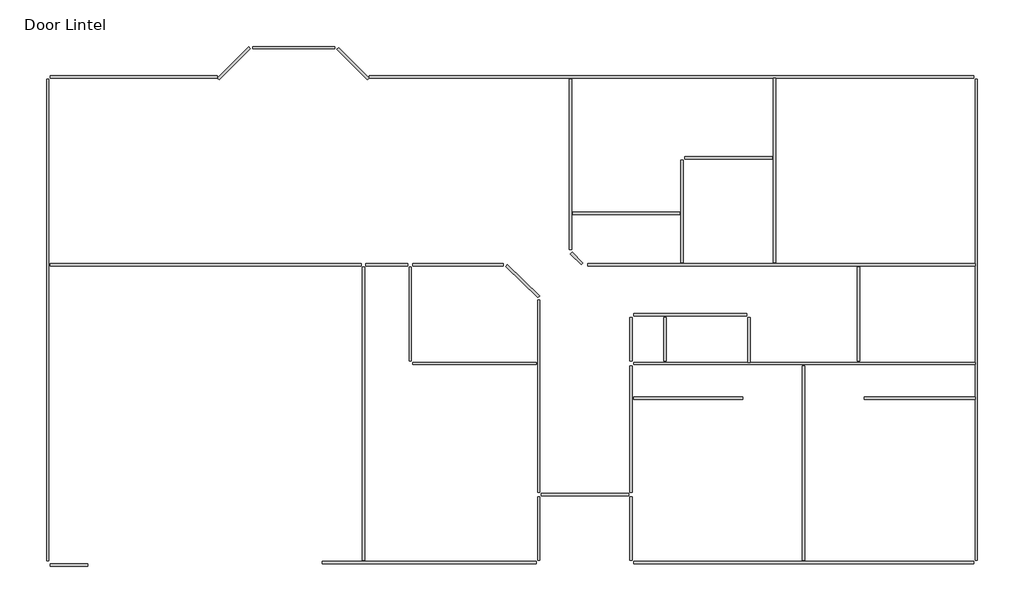
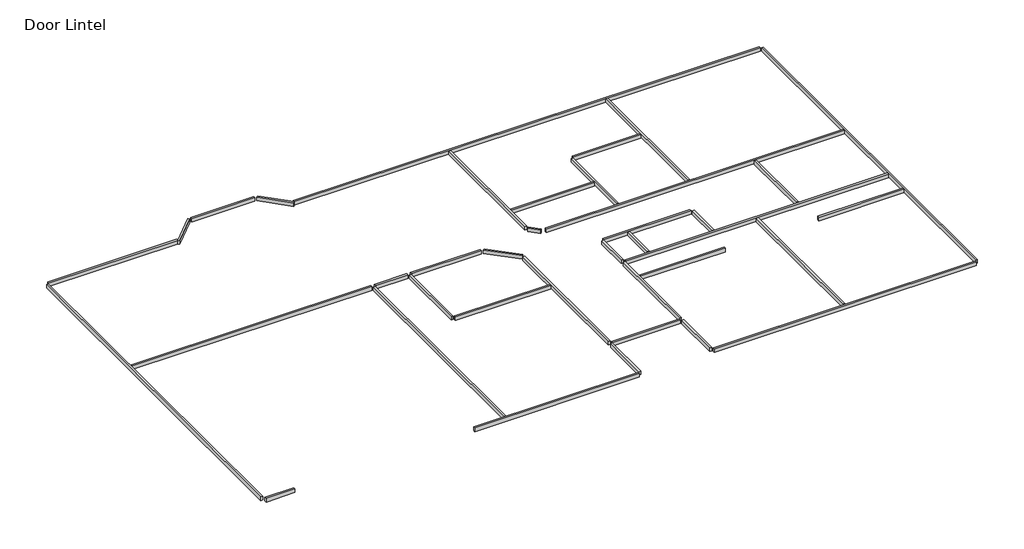
# One storey: 38 beams.
"""IFC4 building model written with IfcOpenShell, lengths in millimetres."""

import ifcopenshell
import ifcopenshell.guid

model = None  # the IFC model being written
_history = None  # IfcOwnerHistory: only IFC2X3 demands one
_inside = {}  # id of a spatial element -> (the spatial element, [elements in it])
_under = {}  # id of a project, library or spatial element -> (it, [spatial elements below it])
_declared = {}  # id of a project -> (the project, [libraries it declares])
_typed = {}  # id of a type object -> (the type object, [elements of that type])
_made_of = {}  # id of a material, layer set ... -> (it, [elements and type objects made of it])


def new_model(schema):
    """Start an empty IFC model of exactly this schema.

    Asked for "IFC4X3", IfcOpenShell would pick the latest addendum, in which some entities
    have other attributes; the version numbers below select the first issue.
    IFC2X3 requires an IfcOwnerHistory on every rooted entity: one is made here for all.
    """
    global model, _history
    if schema == "IFC4X3":
        model = ifcopenshell.file(schema_version=(4, 3, 0, 0))
    else:
        model = ifcopenshell.file(schema=schema)
    _inside.clear()
    _under.clear()
    _declared.clear()
    _typed.clear()
    _made_of.clear()
    _history = None
    if model.schema == "IFC2X3":
        org = make("IfcOrganization", Name="unknown")
        user = make(
            "IfcPersonAndOrganization",
            ThePerson=make("IfcPerson", FamilyName="unknown"),
            TheOrganization=org,
        )
        app = make(
            "IfcApplication",
            ApplicationDeveloper=org,
            Version="unknown",
            ApplicationFullName="unknown",
            ApplicationIdentifier="unknown",
        )
        _history = make(
            "IfcOwnerHistory",
            OwningUser=user,
            OwningApplication=app,
            ChangeAction="ADDED",
            CreationDate=0,
        )
    return model


def make(cls, **values):
    """One entity of the class cls with the attributes given. An attribute that is None is left unset."""
    return model.create_entity(
        cls, **{name: value for name, value in values.items() if value is not None}
    )


def rooted(cls, **values):
    """An entity with a GlobalId (a new one), such as an element, a storey or a relation."""
    return make(cls, GlobalId=ifcopenshell.guid.new(), OwnerHistory=_history, **values)


def si_unit(unit_type, name, prefix=None):
    """IfcSIUnit, for example si_unit("LENGTHUNIT", "METRE", prefix="MILLI")."""
    return make("IfcSIUnit", UnitType=unit_type, Prefix=prefix, Name=name)


def assignment(units):
    """IfcUnitAssignment: the units of a project."""
    return None if units is None else make("IfcUnitAssignment", Units=units)


def point(xyz):
    """IfcCartesianPoint."""
    return None if xyz is None else make("IfcCartesianPoint", Coordinates=xyz)


def direction(xyz):
    """IfcDirection."""
    return None if xyz is None else make("IfcDirection", DirectionRatios=xyz)


def frame(location, z_axis=None, x_axis=None):
    """IfcAxis2Placement3D, a coordinate frame: its origin and axes. An axis left out is left unset."""
    return make(
        "IfcAxis2Placement3D",
        Location=point(location),
        Axis=direction(z_axis),
        RefDirection=direction(x_axis),
    )


def origin():
    """The frame at (0, 0, 0) with its axes left unset."""
    return frame((0.0, 0.0, 0.0))


def place(relative_to, where):
    """IfcLocalPlacement: puts the frame where relative to a parent placement (None: the world)."""
    return make(
        "IfcLocalPlacement", PlacementRelTo=relative_to, RelativePlacement=where
    )


def context(
    kind, dimensions, precision=None, world=None, true_north=None, identifier=None
):
    """IfcGeometricRepresentationContext, for example the 3D "Model" context."""
    return make(
        "IfcGeometricRepresentationContext",
        ContextIdentifier=identifier,
        ContextType=kind,
        CoordinateSpaceDimension=dimensions,
        Precision=precision,
        WorldCoordinateSystem=world,
        TrueNorth=true_north,
    )


def project(units=None, contexts=None):
    """IfcProject with its units and contexts."""
    return rooted(
        "IfcProject",
        Name="project",
        RepresentationContexts=contexts,
        UnitsInContext=assignment(units),
    )


def spatial(cls, under=None, at=None, **own):
    """A site, building, storey or space (cls), placed at a placement, below another one or the project."""
    s = rooted(cls, ObjectPlacement=at, **own)
    if under is not None:
        _under.setdefault(under.id(), (under, []))[1].append(s)
    return s


def polyline(points):
    """IfcPolyline through the points."""
    return make("IfcPolyline", Points=[point(p) for p in points])


def outline(outer, holes=None, kind="AREA"):
    """IfcArbitraryClosedProfileDef: a profile drawn as a closed curve; with holes, ...WithVoids."""
    if holes is None:
        return make("IfcArbitraryClosedProfileDef", ProfileType=kind, OuterCurve=outer)
    return make(
        "IfcArbitraryProfileDefWithVoids",
        ProfileType=kind,
        OuterCurve=outer,
        InnerCurves=holes,
    )


def extrude(swept, where, along, depth):
    """IfcExtrudedAreaSolid: the profile swept, set in the frame where, extruded along a direction by depth."""
    return make(
        "IfcExtrudedAreaSolid",
        SweptArea=swept,
        Position=where,
        ExtrudedDirection=direction(along),
        Depth=depth,
    )


def shape(context_of_items, identifier, shape_type, items):
    """IfcShapeRepresentation: the items that make up one representation, for example the "Body"."""
    return make(
        "IfcShapeRepresentation",
        ContextOfItems=context_of_items,
        RepresentationIdentifier=identifier,
        RepresentationType=shape_type,
        Items=items,
    )


def source(mapping_origin, context_of_items, identifier, shape_type, items):
    """IfcRepresentationMap: a shape defined once, which mapped items show again and again."""
    return make(
        "IfcRepresentationMap",
        MappingOrigin=mapping_origin,
        MappedRepresentation=shape(context_of_items, identifier, shape_type, items),
    )


def transform(
    local_origin,
    x_axis=None,
    y_axis=None,
    z_axis=None,
    scale=None,
    scale2=None,
    scale3=None,
    uniform=True,
):
    """IfcCartesianTransformationOperator3D, or its non-uniform kind. x_axis, y_axis, z_axis: its Axis1, 2, 3."""
    if uniform:
        return make(
            "IfcCartesianTransformationOperator3D",
            Axis1=direction(x_axis),
            Axis2=direction(y_axis),
            LocalOrigin=point(local_origin),
            Scale=scale,
            Axis3=direction(z_axis),
        )
    return make(
        "IfcCartesianTransformationOperator3DnonUniform",
        Axis1=direction(x_axis),
        Axis2=direction(y_axis),
        LocalOrigin=point(local_origin),
        Scale=scale,
        Axis3=direction(z_axis),
        Scale2=scale2,
        Scale3=scale3,
    )


def mapped(mapping_source, mapping_target):
    """IfcMappedItem: shows the shape of a source again, moved by a transform."""
    return make(
        "IfcMappedItem", MappingSource=mapping_source, MappingTarget=mapping_target
    )


def made_of(thing, what):
    """Note that an element or type object is made of a material, layer set ...; save() writes the relation."""
    if what is not None:
        _made_of.setdefault(what.id(), (what, []))[1].append(thing)
    return thing


def element(
    cls,
    number,
    at=None,
    inside=None,
    cuts=None,
    type_object=None,
    material=None,
    context=None,
    identifier="Body",
    shape_type=None,
    held_by="IfcProductDefinitionShape",
    body=None,
    shapes=None,
    **own,
):
    """One element of the class cls, such as IfcWall. Its Tag is "e" and its number.

    at: its placement. inside: the storey or other place that contains it. cuts: it is an
    opening in that element (IfcRelVoidsElement). A single representation is given by context,
    identifier, shape_type and body (its items); several are given by shapes. held_by: the class
    of the entity that holds the representations. save() writes the other relations.
    """
    e = rooted(cls, Tag="e%d" % number, ObjectPlacement=at, **own)
    if body is not None:
        shapes = [shape(context, identifier, shape_type, body)]
    if shapes is not None:
        e.Representation = make(held_by, Representations=shapes)
    if inside is not None:
        _inside.setdefault(inside.id(), (inside, []))[1].append(e)
    if cuts is not None:
        rooted(
            "IfcRelVoidsElement", RelatingBuildingElement=cuts, RelatedOpeningElement=e
        )
    if type_object is not None:
        _typed.setdefault(type_object.id(), (type_object, []))[1].append(e)
    return made_of(e, material)


def aggregate(whole, parts):
    """IfcRelAggregates: a whole, such as a stair, and the parts it consists of."""
    return rooted("IfcRelAggregates", RelatingObject=whole, RelatedObjects=parts)


def save(model, path):
    """Write the relations noted so far, then the file.

    IfcRelAggregates (storeys below a building ...), IfcRelContainedInSpatialStructure (elements
    in a storey), IfcRelDefinesByType, IfcRelAssociatesMaterial and IfcRelDeclares: one each for
    every whole, place, type object, material and project.
    """
    for whole, parts in _under.values():
        aggregate(whole, parts)
    for where, things in _inside.values():
        rooted(
            "IfcRelContainedInSpatialStructure",
            RelatedElements=things,
            RelatingStructure=where,
        )
    for kind, things in _typed.values():
        rooted("IfcRelDefinesByType", RelatedObjects=things, RelatingType=kind)
    for what, things in _made_of.values():
        rooted("IfcRelAssociatesMaterial", RelatedObjects=things, RelatingMaterial=what)
    for by, libraries in _declared.values():
        rooted("IfcRelDeclares", RelatingContext=by, RelatedDefinitions=libraries)
    model.write(path)


def beam_717df711(model_context):
    return source(origin(), model_context, "Body", "SweptSolid", [
        extrude(outline(polyline([(1716.6789755, 25.4), (1716.6789755, -25.4), (-1777.9999994, -25.4), (-1777.9999994, 25.4), (1716.6789755, 25.4)])), frame((0.0, 0.0, -50.8), z_axis=(0.0, 0.0, 1.0), x_axis=(1.0, 0.0, 0.0)), (0.0, 0.0, 1.0), 101.6),
    ])


def beam_0fe92c09(model_context):
    return source(origin(), model_context, "Body", "SweptSolid", [
        extrude(outline(polyline([(431.690501, 25.4), (431.690501, -25.4), (-492.3733183, -25.4), (-492.3733183, 25.4), (431.690501, 25.4)])), frame((0.0, 0.0, -50.8), z_axis=(0.0, 0.0, 1.0), x_axis=(1.0, 0.0, 0.0)), (0.0, 0.0, 1.0), 101.6),
    ])


def beam_3500c81b(model_context):
    return source(origin(), model_context, "Body", "SweptSolid", [
        extrude(outline(polyline([(863.6, 25.4), (863.6, -25.4), (-845.1882072, -25.4), (-845.1882072, 25.4), (863.6, 25.4)])), frame((0.0, 0.0, -50.8), z_axis=(0.0, 0.0, 1.0), x_axis=(1.0, 0.0, 0.0)), (0.0, 0.0, 1.0), 101.6),
    ])


def beam_4e9e3d70(model_context):
    return source(origin(), model_context, "Body", "SweptSolid", [
        extrude(outline(polyline([(492.3733183, 25.4), (492.3733183, -25.4), (-405.6522938, -25.4), (-405.6522938, 25.4), (492.3733183, 25.4)])), frame((0.0, 0.0, -50.8), z_axis=(0.0, 0.0, 1.0), x_axis=(1.0, 0.0, 0.0)), (0.0, 0.0, 1.0), 101.6),
    ])


def beam_5a8d2df6(model_context):
    return source(origin(), model_context, "Body", "SweptSolid", [
        extrude(outline(polyline([(6349.9999994, 25.4), (6349.9999994, -25.4), (-6288.6789755, -25.4), (-6288.6789755, 25.4), (6349.9999994, 25.4)])), frame((0.0, 0.0, -50.8), z_axis=(0.0, 0.0, 1.0), x_axis=(1.0, 0.0, 0.0)), (0.0, 0.0, 1.0), 101.6),
    ])


def beam_8dd97a7c(model_context):
    return source(origin(), model_context, "Body", "SweptSolid", [
        extrude(outline(polyline([(5029.1999994, 25.4), (5029.1999994, -25.4), (-5029.1999994, -25.4), (-5029.1999994, 25.4), (5029.1999994, 25.4)])), frame((0.0, 0.0, -50.8), z_axis=(0.0, 0.0, 1.0), x_axis=(1.0, 0.0, 0.0)), (0.0, 0.0, 1.0), 101.6),
    ])


def beam_44bcd8c2(model_context):
    return source(origin(), model_context, "Body", "SweptSolid", [
        extrude(outline(polyline([(3555.9999994, 25.4), (3555.9999994, -25.4), (-3555.9999994, -25.4), (-3555.9999994, 25.4), (3555.9999994, 25.4)])), frame((0.0, 0.0, -50.8), z_axis=(0.0, 0.0, 1.0), x_axis=(1.0, 0.0, 0.0)), (0.0, 0.0, 1.0), 101.6),
    ])


def beam_ec20356b(model_context):
    return source(origin(), model_context, "Body", "SweptSolid", [
        extrude(outline(polyline([(660.3999994, 25.4), (660.3999994, -25.4), (-660.3999994, -25.4), (-660.3999994, 25.4), (660.3999994, 25.4)])), frame((0.0, 0.0, -50.8), z_axis=(0.0, 0.0, 1.0), x_axis=(1.0, 0.0, 0.0)), (0.0, 0.0, 1.0), 101.6),
    ])


def beam_17170791(model_context):
    return source(origin(), model_context, "Body", "SweptSolid", [
        extrude(outline(polyline([(914.3999994, 25.4), (914.3999994, -25.4), (-914.3999994, -25.4), (-914.3999994, 25.4), (914.3999994, 25.4)])), frame((0.0, 0.0, -50.8), z_axis=(0.0, 0.0, 1.0), x_axis=(1.0, 0.0, 0.0)), (0.0, 0.0, 1.0), 101.6),
    ])


def beam_5c93efd5(model_context):
    return source(origin(), model_context, "Body", "SweptSolid", [
        extrude(outline(polyline([(3063.8749994, 25.4), (3063.8749994, -25.4), (-3063.8749994, -25.4), (-3063.8749994, 25.4), (3063.8749994, 25.4)])), frame((0.0, 0.0, -50.8), z_axis=(0.0, 0.0, 1.0), x_axis=(1.0, 0.0, 0.0)), (0.0, 0.0, 1.0), 101.6),
    ])


def beam_4ff5e491(model_context):
    return source(origin(), model_context, "Body", "SweptSolid", [
        extrude(outline(polyline([(3248.0249994, 25.4), (3248.0249994, -25.4), (-3248.0249994, -25.4), (-3248.0249994, 25.4), (3248.0249994, 25.4)])), frame((0.0, 0.0, -50.8), z_axis=(0.0, 0.0, 1.0), x_axis=(1.0, 0.0, 0.0)), (0.0, 0.0, 1.0), 101.6),
    ])


def beam_e0e1cdb9(model_context):
    return source(origin(), model_context, "Body", "SweptSolid", [
        extrude(outline(polyline([(444.5, 25.4), (444.5, -25.4), (-431.7999994, -25.4), (-431.7999994, 25.4), (444.5, 25.4)])), frame((0.0, 0.0, -50.8), z_axis=(0.0, 0.0, 1.0), x_axis=(1.0, 0.0, 0.0)), (0.0, 0.0, 1.0), 101.6),
    ])


def beam_a7f65a44(model_context):
    return source(origin(), model_context, "Body", "SweptSolid", [
        extrude(outline(polyline([(921.932951, 25.4), (921.932951, -25.4), (-972.7329504, -25.4), (-972.7329504, 25.4), (921.932951, 25.4)])), frame((0.0, 0.0, -50.8), z_axis=(0.0, 0.0, 1.0), x_axis=(1.0, 0.0, 0.0)), (0.0, 0.0, 1.0), 101.6),
    ])


def beam_c7262e2a(model_context):
    return source(origin(), model_context, "Body", "SweptSolid", [
        extrude(outline(polyline([(450.6043361, 25.4), (450.6043361, -25.4), (-488.5308943, -25.4), (-488.5308943, 25.4), (450.6043361, 25.4)])), frame((0.0, 0.0, -50.8), z_axis=(0.0, 0.0, 1.0), x_axis=(1.0, 0.0, 0.0)), (0.0, 0.0, 1.0), 101.6),
    ])


def beam_d1363b41(model_context):
    return source(origin(), model_context, "Body", "SweptSolid", [
        extrude(outline(polyline([(1292.2249994, 25.4), (1292.2249994, -25.4), (-1292.2249994, -25.4), (-1292.2249994, 25.4), (1292.2249994, 25.4)])), frame((0.0, 0.0, -50.8), z_axis=(0.0, 0.0, 1.0), x_axis=(1.0, 0.0, 0.0)), (0.0, 0.0, 1.0), 101.6),
    ])


def beam_1eeaf63e(model_context):
    return source(origin(), model_context, "Body", "SweptSolid", [
        extrude(outline(polyline([(955.675, 25.4), (955.675, -25.4), (-1006.4749994, -25.4), (-1006.4749994, 25.4), (955.675, 25.4)])), frame((0.0, 0.0, -50.8), z_axis=(0.0, 0.0, 1.0), x_axis=(1.0, 0.0, 0.0)), (0.0, 0.0, 1.0), 101.6),
    ])


def beam_6ddf0adc(model_context):
    return source(origin(), model_context, "Body", "SweptSolid", [
        extrude(outline(polyline([(2020.4829504, 25.4), (2020.4829504, -25.4), (-1995.082951, -25.4), (-1995.082951, 25.4), (2020.4829504, 25.4)])), frame((0.0, 0.0, -50.8), z_axis=(0.0, 0.0, 1.0), x_axis=(1.0, 0.0, 0.0)), (0.0, 0.0, 1.0), 101.6),
    ])


def beam_5a6f5897(model_context):
    return source(origin(), model_context, "Body", "SweptSolid", [
        extrude(outline(polyline([(1795.057951, 25.4), (1795.057951, -25.4), (-1769.657951, -25.4), (-1769.657951, 25.4), (1795.057951, 25.4)])), frame((0.0, 0.0, -50.8), z_axis=(0.0, 0.0, 1.0), x_axis=(1.0, 0.0, 0.0)), (0.0, 0.0, 1.0), 101.6),
    ])


def beam_8933aaf6(model_context):
    return source(origin(), model_context, "Body", "SweptSolid", [
        extrude(outline(polyline([(161.5124332, 25.4), (161.5124332, -25.4), (-161.5124332, -25.4), (-161.5124332, 25.4), (161.5124332, 25.4)])), frame((0.0, 0.0, -50.8), z_axis=(0.0, 0.0, 1.0), x_axis=(1.0, 0.0, 0.0)), (0.0, 0.0, 1.0), 101.6),
    ])


def beam_50604119(model_context):
    return source(origin(), model_context, "Body", "SweptSolid", [
        extrude(outline(polyline([(1117.6, 25.4), (1117.6, -25.4), (-1117.6, -25.4), (-1117.6, 25.4), (1117.6, 25.4)])), frame((0.0, 0.0, -50.8), z_axis=(0.0, 0.0, 1.0), x_axis=(1.0, 0.0, 0.0)), (0.0, 0.0, 1.0), 101.6),
    ])


def beam_0149d91d(model_context):
    return source(origin(), model_context, "Body", "SweptSolid", [
        extrude(outline(polyline([(4058.832951, 25.4), (4058.832951, -25.4), (-4033.432951, -25.4), (-4033.432951, 25.4), (4058.832951, 25.4)])), frame((0.0, 0.0, -50.8), z_axis=(0.0, 0.0, 1.0), x_axis=(1.0, 0.0, 0.0)), (0.0, 0.0, 1.0), 101.6),
    ])


def beam_4f4e5714(model_context):
    return source(origin(), model_context, "Body", "SweptSolid", [
        extrude(outline(polyline([(1066.8, 25.4), (1066.8, -25.4), (-1066.8, -25.4), (-1066.8, 25.4), (1066.8, 25.4)])), frame((0.0, 0.0, -50.8), z_axis=(0.0, 0.0, 1.0), x_axis=(1.0, 0.0, 0.0)), (0.0, 0.0, 1.0), 101.6),
    ])


def beam_dc030418(model_context):
    return source(origin(), model_context, "Body", "SweptSolid", [
        extrude(outline(polyline([(914.4, 25.4), (914.4, -25.4), (-914.4, -25.4), (-914.4, 25.4), (914.4, 25.4)])), frame((0.0, 0.0, -50.8), z_axis=(0.0, 0.0, 1.0), x_axis=(1.0, 0.0, 0.0)), (0.0, 0.0, 1.0), 101.6),
    ])


def beam_32b3ca21(model_context):
    return source(origin(), model_context, "Body", "SweptSolid", [
        extrude(outline(polyline([(1914.525, 25.4), (1914.525, -25.4), (-1939.925, -25.4), (-1939.925, 25.4), (1914.525, 25.4)])), frame((0.0, 0.0, -50.8), z_axis=(0.0, 0.0, 1.0), x_axis=(1.0, 0.0, 0.0)), (0.0, 0.0, 1.0), 101.6),
    ])


def beam_af15350c(model_context):
    return source(origin(), model_context, "Body", "SweptSolid", [
        extrude(outline(polyline([(1181.1, 25.4), (1181.1, -25.4), (-1181.1, -25.4), (-1181.1, 25.4), (1181.1, 25.4)])), frame((0.0, 0.0, -50.8), z_axis=(0.0, 0.0, 1.0), x_axis=(1.0, 0.0, 0.0)), (0.0, 0.0, 1.0), 101.6),
    ])


def beam_60fbd3f3(model_context):
    return source(origin(), model_context, "Body", "SweptSolid", [
        extrude(outline(polyline([(457.2, 25.4), (457.2, -25.4), (-457.2, -25.4), (-457.2, 25.4), (457.2, 25.4)])), frame((0.0, 0.0, -50.8), z_axis=(0.0, 0.0, 1.0), x_axis=(1.0, 0.0, 0.0)), (0.0, 0.0, 1.0), 101.6),
    ])


def beam_38f3c654(model_context):
    return source(origin(), model_context, "Body", "SweptSolid", [
        extrude(outline(polyline([(3581.4, 25.4), (3581.4, -25.4), (-3556.0, -25.4), (-3556.0, 25.4), (3581.4, 25.4)])), frame((0.0, 0.0, -50.8), z_axis=(0.0, 0.0, 1.0), x_axis=(1.0, 0.0, 0.0)), (0.0, 0.0, 1.0), 101.6),
    ])


def beam_f72471f4(model_context):
    return source(origin(), model_context, "Body", "SweptSolid", [
        extrude(outline(polyline([(482.6, 25.4), (482.6, -25.4), (-457.2, -25.4), (-457.2, 25.4), (482.6, 25.4)])), frame((0.0, 0.0, -50.8), z_axis=(0.0, 0.0, 1.0), x_axis=(1.0, 0.0, 0.0)), (0.0, 0.0, 1.0), 101.6),
    ])


def beam_0b80d38c(model_context):
    return source(origin(), model_context, "Body", "SweptSolid", [
        extrude(outline(polyline([(1143.0, 25.4), (1143.0, -25.4), (-1143.0, -25.4), (-1143.0, 25.4), (1143.0, 25.4)])), frame((0.0, 0.0, -50.8), z_axis=(0.0, 0.0, 1.0), x_axis=(1.0, 0.0, 0.0)), (0.0, 0.0, 1.0), 101.6),
    ])


def beam_8729cf3f(model_context):
    return source(origin(), model_context, "Body", "SweptSolid", [
        extrude(outline(polyline([(981.075, 25.4), (981.075, -25.4), (-981.075, -25.4), (-981.075, 25.4), (981.075, 25.4)])), frame((0.0, 0.0, -50.8), z_axis=(0.0, 0.0, 1.0), x_axis=(1.0, 0.0, 0.0)), (0.0, 0.0, 1.0), 101.6),
    ])


def beam_71e3b4ab(model_context):
    return source(origin(), model_context, "Body", "SweptSolid", [
        extrude(outline(polyline([(1168.4, 25.4), (1168.4, -25.4), (-1143.0, -25.4), (-1143.0, 25.4), (1168.4, 25.4)])), frame((0.0, 0.0, -50.8), z_axis=(0.0, 0.0, 1.0), x_axis=(1.0, 0.0, 0.0)), (0.0, 0.0, 1.0), 101.6),
    ])


def beam_d87feb12(model_context):
    return source(origin(), model_context, "Body", "SweptSolid", [
        extrude(outline(polyline([(2032.0, 25.4), (2032.0, -25.4), (-2032.0, -25.4), (-2032.0, 25.4), (2032.0, 25.4)])), frame((0.0, 0.0, -50.8), z_axis=(0.0, 0.0, 1.0), x_axis=(1.0, 0.0, 0.0)), (0.0, 0.0, 1.0), 101.6),
    ])


def beam_35a73032(model_context):
    return source(origin(), model_context, "Body", "SweptSolid", [
        extrude(outline(polyline([(1320.8, 25.4), (1320.8, -25.4), (-1320.8, -25.4), (-1320.8, 25.4), (1320.8, 25.4)])), frame((0.0, 0.0, -50.8), z_axis=(0.0, 0.0, 1.0), x_axis=(1.0, 0.0, 0.0)), (0.0, 0.0, 1.0), 101.6),
    ])


def beam_ce158ae4(model_context):
    return source(origin(), model_context, "Body", "SweptSolid", [
        extrude(outline(polyline([(392.1124994, 25.4), (392.1124994, -25.4), (-392.1125, -25.4), (-392.1125, 25.4), (392.1124994, 25.4)])), frame((0.0, 0.0, -50.8), z_axis=(0.0, 0.0, 1.0), x_axis=(1.0, 0.0, 0.0)), (0.0, 0.0, 1.0), 101.6),
    ])


def beam_4f005310(model_context):
    return source(origin(), model_context, "Body", "SweptSolid", [
        extrude(outline(polyline([(5035.5499994, 25.4), (5035.5499994, -25.4), (-5035.55, -25.4), (-5035.55, 25.4), (5035.5499994, 25.4)])), frame((0.0, 0.0, -50.8), z_axis=(0.0, 0.0, 1.0), x_axis=(1.0, 0.0, 0.0)), (0.0, 0.0, 1.0), 101.6),
    ])


def beam_f884bc05(model_context):
    return source(origin(), model_context, "Body", "SweptSolid", [
        extrude(outline(polyline([(2235.2, 25.4), (2235.2, -25.4), (-2235.1999994, -25.4), (-2235.1999994, 25.4), (2235.2, 25.4)])), frame((0.0, 0.0, -50.8), z_axis=(0.0, 0.0, 1.0), x_axis=(1.0, 0.0, 0.0)), (0.0, 0.0, 1.0), 101.6),
    ])


model = new_model("IFC4")

# Units and contexts
model_context = context("Model", 3, world=origin())
ifc_project = project(units=[si_unit("LENGTHUNIT", "METRE", prefix="MILLI")], contexts=[model_context])

# Site, building, storey
site = spatial("IfcSite", under=ifc_project)
building = spatial("IfcBuilding", under=site)
storey = spatial("IfcBuildingStorey", under=building, Name="Door Lintel", Elevation=2387.6)

# Beams
placement = place(None, origin())
beam_shape = beam_717df711(model_context)
element("IfcBeam", 1, ObjectType="Dimension Lumber : BLDG 6241 2X4\" TRUSS MEMBER", at=placement, inside=storey, context=model_context, shape_type="MappedRepresentation", body=[
    mapped(beam_shape, transform((-15921.614829, 5156.9284114, 2336.8), x_axis=(1.0, 0.0, 0.0), y_axis=(0.0, 1.0, 0.0), z_axis=(0.0, 0.0, 1.0))),
])
beam_2_shape = beam_0fe92c09(model_context)
element("IfcBeam", 2, ObjectType="Dimension Lumber : BLDG 6241 2X4\" TRUSS MEMBER", at=placement, inside=storey, context=model_context, shape_type="MappedRepresentation", body=[
    mapped(beam_2_shape, transform((-13838.814829, 5461.7284114, 2336.8), x_axis=(0.7071067811865482, 0.7071067811865469, 0.0), y_axis=(-0.7071067811865469, 0.7071067811865482, 0.0), z_axis=(0.0, 0.0, 1.0))),
])
beam_3_shape = beam_3500c81b(model_context)
element("IfcBeam", 3, ObjectType="Dimension Lumber : BLDG 6241 2X4\" TRUSS MEMBER", at=placement, inside=storey, context=model_context, shape_type="MappedRepresentation", body=[
    mapped(beam_3_shape, transform((-12619.614829, 5766.5284114, 2336.8), x_axis=(1.0, 0.0, 0.0), y_axis=(0.0, 1.0, 0.0), z_axis=(0.0, 0.0, 1.0))),
])
beam_4_shape = beam_4e9e3d70(model_context)
element("IfcBeam", 4, ObjectType="Dimension Lumber : BLDG 6241 2X4\" TRUSS MEMBER", at=placement, inside=storey, context=model_context, shape_type="MappedRepresentation", body=[
    mapped(beam_4_shape, transform((-11400.414829, 5461.7284114, 2336.8), x_axis=(0.7071067811865464, -0.7071067811865488, 0.0), y_axis=(0.7071067811865488, 0.7071067811865464, 0.0), z_axis=(0.0, 0.0, 1.0))),
])
beam_5_shape = beam_5a8d2df6(model_context)
element("IfcBeam", 5, ObjectType="Dimension Lumber : BLDG 6241 2X4\" TRUSS MEMBER", at=placement, inside=storey, context=model_context, shape_type="MappedRepresentation", body=[
    mapped(beam_5_shape, transform((-4745.614829, 5156.9284114, 2336.8), x_axis=(1.0, 0.0, 0.0), y_axis=(0.0, 1.0, 0.0), z_axis=(0.0, 0.0, 1.0))),
])
beam_6_shape = beam_8dd97a7c(model_context)
element("IfcBeam", 6, ObjectType="Dimension Lumber : BLDG 6241 2X4\" TRUSS MEMBER", at=placement, inside=storey, context=model_context, shape_type="MappedRepresentation", body=[
    mapped(beam_6_shape, transform((1655.185171, 76.9284114, 2336.8), x_axis=(0.0, -1.0, 0.0), y_axis=(1.0, 0.0, 0.0), z_axis=(0.0, 0.0, 1.0))),
])
beam_7_shape = beam_44bcd8c2(model_context)
element("IfcBeam", 7, ObjectType="Dimension Lumber : BLDG 6241 2X4\" TRUSS MEMBER", at=placement, inside=storey, context=model_context, shape_type="MappedRepresentation", body=[
    mapped(beam_7_shape, transform((-1951.614829, -5003.0715886, 2336.8), x_axis=(-1.0, 0.0, 0.0), y_axis=(0.0, -1.0, 0.0), z_axis=(0.0, 0.0, 1.0))),
])
beam_8_shape = beam_ec20356b(model_context)
element("IfcBeam", 8, ObjectType="Dimension Lumber : BLDG 6241 2X4\" TRUSS MEMBER", at=placement, inside=storey, context=model_context, shape_type="MappedRepresentation", body=[
    mapped(beam_8_shape, transform((-5558.414829, -4291.8715886, 2336.8), x_axis=(0.0, 1.0, 0.0), y_axis=(-1.0, 0.0, 0.0), z_axis=(0.0, 0.0, 1.0))),
])
element("IfcBeam", 9, ObjectType="Dimension Lumber : BLDG 6241 2X4\" TRUSS MEMBER", at=placement, inside=storey, context=model_context, shape_type="MappedRepresentation", body=[
    mapped(beam_8_shape, transform((-7488.814829, -4291.8715886, 2336.8), x_axis=(0.0, -1.0, 0.0), y_axis=(1.0, 0.0, 0.0), z_axis=(0.0, 0.0, 1.0))),
])
beam_9_shape = beam_17170791(model_context)
element("IfcBeam", 10, ObjectType="Dimension Lumber : BLDG 6241 2X4\" TRUSS MEMBER", at=placement, inside=storey, context=model_context, shape_type="MappedRepresentation", body=[
    mapped(beam_9_shape, transform((-6523.614829, -3580.6715886, 2336.8), x_axis=(-1.0, 0.0, 0.0), y_axis=(0.0, -1.0, 0.0), z_axis=(0.0, 0.0, 1.0))),
])
beam_10_shape = beam_5c93efd5(model_context)
element("IfcBeam", 11, ObjectType="Dimension Lumber : BLDG 6241 2X4\" TRUSS MEMBER", at=placement, inside=storey, context=model_context, shape_type="MappedRepresentation", body=[
    mapped(beam_10_shape, transform((-11152.764829, -1888.3965886, 2336.8), x_axis=(0.0, 1.0, 0.0), y_axis=(-1.0, 0.0, 0.0), z_axis=(0.0, 0.0, 1.0))),
])
beam_11_shape = beam_4ff5e491(model_context)
element("IfcBeam", 12, ObjectType="Dimension Lumber : BLDG 6241 2X4\" TRUSS MEMBER", at=placement, inside=storey, context=model_context, shape_type="MappedRepresentation", body=[
    mapped(beam_11_shape, transform((-14451.589829, 1226.2784114, 2336.8), x_axis=(-1.0, 0.0, 0.0), y_axis=(0.0, -1.0, 0.0), z_axis=(0.0, 0.0, 1.0))),
])
beam_12_shape = beam_e0e1cdb9(model_context)
element("IfcBeam", 13, ObjectType="Dimension Lumber : BLDG 6241 2X4\" TRUSS MEMBER", at=placement, inside=storey, context=model_context, shape_type="MappedRepresentation", body=[
    mapped(beam_12_shape, transform((-10670.164829, 1226.2784114, 2336.8), x_axis=(1.0, 0.0, 0.0), y_axis=(0.0, 1.0, 0.0), z_axis=(0.0, 0.0, 1.0))),
])
beam_13_shape = beam_a7f65a44(model_context)
element("IfcBeam", 14, ObjectType="Dimension Lumber : BLDG 6241 2X4\" TRUSS MEMBER", at=placement, inside=storey, context=model_context, shape_type="MappedRepresentation", body=[
    mapped(beam_13_shape, transform((-9151.331878, 1226.2784114, 2336.8), x_axis=(1.0, 0.0, 0.0), y_axis=(0.0, 1.0, 0.0), z_axis=(0.0, 0.0, 1.0))),
])
beam_14_shape = beam_c7262e2a(model_context)
element("IfcBeam", 15, ObjectType="Dimension Lumber : BLDG 6241 2X4\" TRUSS MEMBER", at=placement, inside=storey, context=model_context, shape_type="MappedRepresentation", body=[
    mapped(beam_14_shape, transform((-7810.4858535, 868.6863624, 2336.8), x_axis=(0.7172827972504613, -0.6967821673726686, 0.0), y_axis=(0.6967821673726686, 0.7172827972504613, 0.0), z_axis=(0.0, 0.0, 1.0))),
])
beam_15_shape = beam_d1363b41(model_context)
element("IfcBeam", 16, ObjectType="Dimension Lumber : BLDG 6241 2X4\" TRUSS MEMBER", at=placement, inside=storey, context=model_context, shape_type="MappedRepresentation", body=[
    mapped(beam_15_shape, transform((-8831.839829, -837.4715886, 2336.8), x_axis=(1.0, 0.0, 0.0), y_axis=(0.0, 1.0, 0.0), z_axis=(0.0, 0.0, 1.0))),
])
beam_16_shape = beam_1eeaf63e(model_context)
element("IfcBeam", 17, ObjectType="Dimension Lumber : BLDG 6241 2X4\" TRUSS MEMBER", at=placement, inside=storey, context=model_context, shape_type="MappedRepresentation", body=[
    mapped(beam_16_shape, transform((-10174.864829, 219.8034114, 2336.8), x_axis=(0.0, 1.0, 0.0), y_axis=(-1.0, 0.0, 0.0), z_axis=(0.0, 0.0, 1.0))),
])
beam_17_shape = beam_6ddf0adc(model_context)
element("IfcBeam", 18, ObjectType="Dimension Lumber : BLDG 6241 2X4\" TRUSS MEMBER", at=placement, inside=storey, context=model_context, shape_type="MappedRepresentation", body=[
    mapped(beam_17_shape, transform((-7488.814829, -1509.3886376, 2336.8), x_axis=(0.0, -1.0, 0.0), y_axis=(1.0, 0.0, 0.0), z_axis=(0.0, 0.0, 1.0))),
])
beam_18_shape = beam_5a6f5897(model_context)
element("IfcBeam", 19, ObjectType="Dimension Lumber : BLDG 6241 2X4\" TRUSS MEMBER", at=placement, inside=storey, context=model_context, shape_type="MappedRepresentation", body=[
    mapped(beam_18_shape, transform((-6828.414829, 3336.4704603, 2336.8), x_axis=(0.0, -1.0, 0.0), y_axis=(1.0, 0.0, 0.0), z_axis=(0.0, 0.0, 1.0))),
])
beam_19_shape = beam_8933aaf6(model_context)
element("IfcBeam", 20, ObjectType="Dimension Lumber : BLDG 6241 2X4\" TRUSS MEMBER", at=placement, inside=storey, context=model_context, shape_type="MappedRepresentation", body=[
    mapped(beam_19_shape, transform((-6696.2477801, 1358.4454603, 2336.8), x_axis=(-0.7071067811865457, 0.7071067811865493, 0.0), y_axis=(-0.7071067811865493, -0.7071067811865457, 0.0), z_axis=(0.0, 0.0, 1.0))),
])
beam_20_shape = beam_50604119(model_context)
element("IfcBeam", 21, ObjectType="Dimension Lumber : BLDG 6241 2X4\" TRUSS MEMBER", at=placement, inside=storey, context=model_context, shape_type="MappedRepresentation", body=[
    mapped(beam_20_shape, transform((-5660.014829, 2305.7784114, 2336.8), x_axis=(1.0, 0.0, 0.0), y_axis=(0.0, 1.0, 0.0), z_axis=(0.0, 0.0, 1.0))),
])
beam_21_shape = beam_0149d91d(model_context)
element("IfcBeam", 22, ObjectType="Dimension Lumber : BLDG 6241 2X4\" TRUSS MEMBER", at=placement, inside=storey, context=model_context, shape_type="MappedRepresentation", body=[
    mapped(beam_21_shape, transform((-2429.0477801, 1226.2784114, 2336.8), x_axis=(1.0, 0.0, 0.0), y_axis=(0.0, 1.0, 0.0), z_axis=(0.0, 0.0, 1.0))),
])
beam_22_shape = beam_4f4e5714(model_context)
element("IfcBeam", 23, ObjectType="Dimension Lumber : BLDG 6241 2X4\" TRUSS MEMBER", at=placement, inside=storey, context=model_context, shape_type="MappedRepresentation", body=[
    mapped(beam_22_shape, transform((-4491.614829, 2343.8784114, 2336.8), x_axis=(0.0, 1.0, 0.0), y_axis=(-1.0, 0.0, 0.0), z_axis=(0.0, 0.0, 1.0))),
])
beam_23_shape = beam_dc030418(model_context)
element("IfcBeam", 24, ObjectType="Dimension Lumber : BLDG 6241 2X4\" TRUSS MEMBER", at=placement, inside=storey, context=model_context, shape_type="MappedRepresentation", body=[
    mapped(beam_23_shape, transform((-3526.414829, 3461.4784114, 2336.8), x_axis=(1.0, 0.0, 0.0), y_axis=(0.0, 1.0, 0.0), z_axis=(0.0, 0.0, 1.0))),
])
beam_24_shape = beam_32b3ca21(model_context)
element("IfcBeam", 25, ObjectType="Dimension Lumber : BLDG 6241 2X4\" TRUSS MEMBER", at=placement, inside=storey, context=model_context, shape_type="MappedRepresentation", body=[
    mapped(beam_24_shape, transform((-2561.214829, 3191.6034114, 2336.8), x_axis=(0.0, -1.0, 0.0), y_axis=(1.0, 0.0, 0.0), z_axis=(0.0, 0.0, 1.0))),
])
beam_25_shape = beam_af15350c(model_context)
element("IfcBeam", 26, ObjectType="Dimension Lumber : BLDG 6241 2X4\" TRUSS MEMBER", at=placement, inside=storey, context=model_context, shape_type="MappedRepresentation", body=[
    mapped(beam_25_shape, transform((-4326.514829, 178.5284114, 2336.8), x_axis=(1.0, 0.0, 0.0), y_axis=(0.0, 1.0, 0.0), z_axis=(0.0, 0.0, 1.0))),
])
beam_26_shape = beam_60fbd3f3(model_context)
element("IfcBeam", 27, ObjectType="Dimension Lumber : BLDG 6241 2X4\" TRUSS MEMBER", at=placement, inside=storey, context=model_context, shape_type="MappedRepresentation", body=[
    mapped(beam_26_shape, transform((-5558.414829, -329.4715886, 2336.8), x_axis=(0.0, 1.0, 0.0), y_axis=(-1.0, 0.0, 0.0), z_axis=(0.0, 0.0, 1.0))),
])
element("IfcBeam", 28, ObjectType="Dimension Lumber : BLDG 6241 2X4\" TRUSS MEMBER", at=placement, inside=storey, context=model_context, shape_type="MappedRepresentation", body=[
    mapped(beam_26_shape, transform((-4847.214829, -329.4715886, 2336.8), x_axis=(0.0, 1.0, 0.0), y_axis=(-1.0, 0.0, 0.0), z_axis=(0.0, 0.0, 1.0))),
])
beam_27_shape = beam_38f3c654(model_context)
element("IfcBeam", 29, ObjectType="Dimension Lumber : BLDG 6241 2X4\" TRUSS MEMBER", at=placement, inside=storey, context=model_context, shape_type="MappedRepresentation", body=[
    mapped(beam_27_shape, transform((-1951.614829, -837.4715886, 2336.8), x_axis=(1.0, 0.0, 0.0), y_axis=(0.0, 1.0, 0.0), z_axis=(0.0, 0.0, 1.0))),
])
beam_28_shape = beam_f72471f4(model_context)
element("IfcBeam", 30, ObjectType="Dimension Lumber : BLDG 6241 2X4\" TRUSS MEMBER", at=placement, inside=storey, context=model_context, shape_type="MappedRepresentation", body=[
    mapped(beam_28_shape, transform((-3094.614829, -329.4715886, 2336.8), x_axis=(0.0, -1.0, 0.0), y_axis=(1.0, 0.0, 0.0), z_axis=(0.0, 0.0, 1.0))),
])
beam_29_shape = beam_0b80d38c(model_context)
element("IfcBeam", 31, ObjectType="Dimension Lumber : BLDG 6241 2X4\" TRUSS MEMBER", at=placement, inside=storey, context=model_context, shape_type="MappedRepresentation", body=[
    mapped(beam_29_shape, transform((-4364.614829, -1561.3715886, 2336.8), x_axis=(1.0, 0.0, 0.0), y_axis=(0.0, 1.0, 0.0), z_axis=(0.0, 0.0, 1.0))),
])
beam_30_shape = beam_8729cf3f(model_context)
element("IfcBeam", 32, ObjectType="Dimension Lumber : BLDG 6241 2X4\" TRUSS MEMBER", at=placement, inside=storey, context=model_context, shape_type="MappedRepresentation", body=[
    mapped(beam_30_shape, transform((-808.614829, 194.4034114, 2336.8), x_axis=(0.0, -1.0, 0.0), y_axis=(1.0, 0.0, 0.0), z_axis=(0.0, 0.0, 1.0))),
])
beam_31_shape = beam_71e3b4ab(model_context)
element("IfcBeam", 33, ObjectType="Dimension Lumber : BLDG 6241 2X4\" TRUSS MEMBER", at=placement, inside=storey, context=model_context, shape_type="MappedRepresentation", body=[
    mapped(beam_31_shape, transform((461.385171, -1561.3715886, 2336.8), x_axis=(1.0, 0.0, 0.0), y_axis=(0.0, 1.0, 0.0), z_axis=(0.0, 0.0, 1.0))),
])
beam_32_shape = beam_d87feb12(model_context)
element("IfcBeam", 34, ObjectType="Dimension Lumber : BLDG 6241 2X4\" TRUSS MEMBER", at=placement, inside=storey, context=model_context, shape_type="MappedRepresentation", body=[
    mapped(beam_32_shape, transform((-1951.614829, -2920.2715886, 2336.8), x_axis=(0.0, 1.0, 0.0), y_axis=(-1.0, 0.0, 0.0), z_axis=(0.0, 0.0, 1.0))),
])
beam_33_shape = beam_35a73032(model_context)
element("IfcBeam", 35, ObjectType="Dimension Lumber : BLDG 6241 2X4\" TRUSS MEMBER", at=placement, inside=storey, context=model_context, shape_type="MappedRepresentation", body=[
    mapped(beam_33_shape, transform((-5558.414829, -2209.0715886, 2336.8), x_axis=(0.0, 1.0, 0.0), y_axis=(-1.0, 0.0, 0.0), z_axis=(0.0, 0.0, 1.0))),
])
beam_34_shape = beam_ce158ae4(model_context)
element("IfcBeam", 36, ObjectType="Dimension Lumber : BLDG 6241 2X4\" TRUSS MEMBER", at=placement, inside=storey, context=model_context, shape_type="MappedRepresentation", body=[
    mapped(beam_34_shape, transform((-17307.502329, -5053.8715886, 2336.8), x_axis=(-1.0, 0.0, 0.0), y_axis=(0.0, -1.0, 0.0), z_axis=(0.0, 0.0, 1.0))),
])
beam_35_shape = beam_4f005310(model_context)
element("IfcBeam", 37, ObjectType="Dimension Lumber : BLDG 6241 2X4\" TRUSS MEMBER", at=placement, inside=storey, context=model_context, shape_type="MappedRepresentation", body=[
    mapped(beam_35_shape, transform((-17750.414829, 70.5784114, 2336.8), x_axis=(0.0, 1.0, 0.0), y_axis=(-1.0, 0.0, 0.0), z_axis=(0.0, 0.0, 1.0))),
])
beam_36_shape = beam_f884bc05(model_context)
element("IfcBeam", 38, ObjectType="Dimension Lumber : BLDG 6241 2X4\" TRUSS MEMBER", at=placement, inside=storey, context=model_context, shape_type="MappedRepresentation", body=[
    mapped(beam_36_shape, transform((-9774.814829, -5003.0715886, 2336.8), x_axis=(-1.0, 0.0, 0.0), y_axis=(0.0, -1.0, 0.0), z_axis=(0.0, 0.0, 1.0))),
])

save(model, "model.ifc")

# Revit data of these elements
# Type "Dimension Lumber : BLDG 6241 2X4\" TRUSS MEMBER"
#   Assembly Code = "B10"
#   A = 0.273472 SF
#   Length [instance default] = 5' - 0"
#   b = 0' - 2"
#   d = 0' - 4"
#   Structural Material [instance default] = Softwood, Lumber
# Elements 1, 2, 3, 4, 5, 6, 7, 8, 9, 10, 11, 12, 13, 14, 15, 16, 17, 18, 19, 20, 21, 22, 23, 24, 25, 26, 27, 28, 29, 30, 31, 32, 33, 34, 35, 36, 37, 38 (IfcBeam, "Dimension Lumber : BLDG 6241 2X4\" TRUSS MEMBER")
#   Comments = ""
#   Structural Material = Softwood, Lumber
#   Phase Created = New Construction
#   Materials on its faces: "Softwood, Lumber"
# Materials
#   "Softwood, Lumber": class "Wood", colour RGB 223 192 134, transparency 0, Description = "Pinus Echinata", Cost = 0
